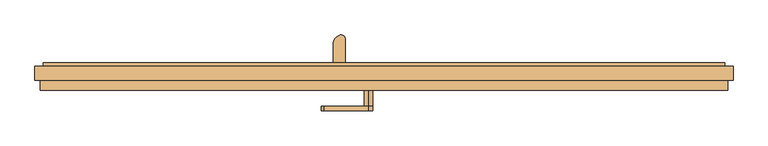
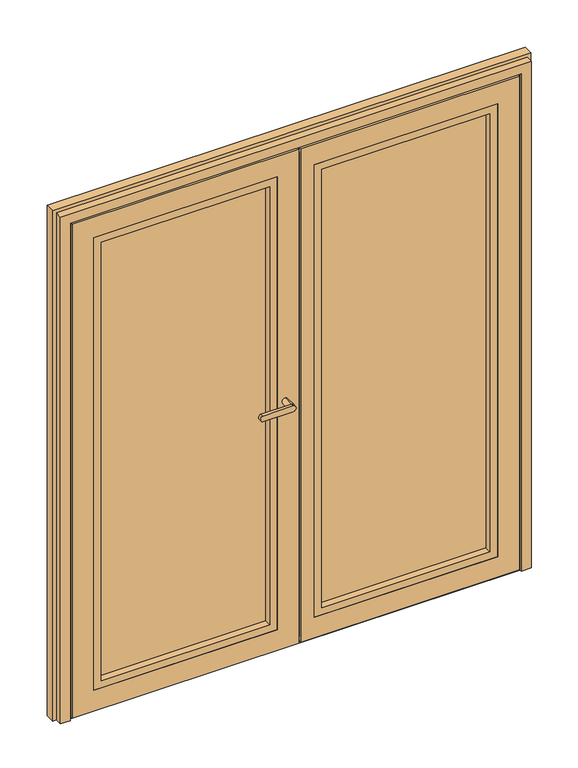
"""IFC4 building model written with IfcOpenShell, lengths in millimetres: door geometry, Schueco_FWS_ADS-75-SimplySmart_inw_Family-02 : FWS SI insert unit."""

from ifc_helpers import new_model, si_unit, point, frame, frame_2d, origin, place, context, project, spatial, polyline, circle_curve, ellipse_curve, trimmed, segment, composite_curve, outline, extrude, faceted_brep, source, transform, mapped, element, save
from ifc_brep_helpers import plane_surface, cylinder_surface, extruded_surface, advanced_brep


def door_de44d966(model_context):
    return source(origin(), model_context, "Body", "SolidModel", [
        faceted_brep([(893.0, -57.5000065, 8.0), (893.0, -57.5000065, 2093.0), (893.0, -66.0002823, 2093.0), (893.0, -66.0002823, 8.0), (19.5, -66.0002823, 8.0), (19.5, -57.5000065, 8.0), (19.5, -57.5000065, 27.0), (874.0, -57.5000065, 27.0), (874.0, -57.5000065, 2074.0), (19.5, -57.5000065, 2074.0), (19.5, -57.5000065, 2093.0), (19.5, -66.0002823, 2093.0), (74.5, -66.0002823, 95.0), (74.5, -66.0002823, 2006.0), (806.0, -66.0002823, 2006.0), (806.0, -66.0002823, 95.0), (806.0, 0.4997603, 2006.0), (806.0, 0.4997603, 95.0), (74.5, 0.4997603, 95.0), (74.5, 0.4997603, 2006.0), (106.5, 0.4997603, 127.0), (106.5, 0.4997603, 1974.0), (774.0, 0.4997603, 1974.0), (774.0, 0.4997603, 127.0), (774.0, 8.9997177, 1974.0), (774.0, 8.9997177, 127.0), (106.5, 8.9997177, 127.0), (106.5, 8.9997177, 1974.0), (861.0, 8.9997177, 40.0), (-12.5, 8.9997177, 40.0), (-12.5, 8.9997177, 2061.0), (861.0, 8.9997177, 2061.0), (861.0, 0.4997603, 2061.0), (861.0, 0.4997603, 40.0), (6.5, 0.4997603, 40.0), (-12.5, 0.4997603, 40.0), (6.5, 0.4997603, 27.0), (6.5, 0.4997603, 2061.0), (6.5, 0.4997603, 2074.0), (874.0, 0.4997603, 2074.0), (874.0, 0.4997603, 27.0), (6.5, -57.5000065, 27.0), (6.5, -57.5000065, 2074.0), (-12.5, 0.4997603, 2061.0)], [[[0, 1, 2, 3]], [[3, 4, 5, 0]], [[0, 5, 6, 7, 8, 9, 10, 1]], [[2, 11, 4, 3], [12, 13, 14, 15]], [[15, 14, 16, 17]], [[17, 18, 12, 15]], [[18, 19, 13, 12]], [[17, 16, 19, 18], [20, 21, 22, 23]], [[23, 22, 24, 25]], [[25, 26, 20, 23]], [[26, 27, 21, 20]], [[28, 29, 30, 31], [25, 24, 27, 26]], [[28, 31, 32, 33]], [[33, 34, 35, 29, 28]], [[36, 34, 33, 32, 37, 38, 39, 40]], [[40, 39, 8, 7]], [[7, 6, 41, 36, 40]], [[41, 42, 38, 37, 34, 36]], [[1, 10, 11, 2]], [[19, 16, 14, 13]], [[27, 24, 22, 21]], [[31, 30, 43, 37, 32]], [[42, 9, 8, 39, 38]], [[6, 5, 4, 11, 10, 9]], [[35, 43, 30, 29]], [[35, 34, 37, 43]], [[9, 42, 41, 6]]]),
        extrude(outline(polyline([(95.0, 74.5), (95.0, 806.0), (2006.0, 806.0), (2006.0, 74.5), (95.0, 74.5)]), holes=[polyline([(125.0, 776.0), (125.0, 104.5), (1976.0, 104.5), (1976.0, 776.0), (125.0, 776.0)])]), frame((0.0, -66.0002823, 0.0), z_axis=(0.0, 1.0, 0.0), x_axis=(0.0, 0.0, 1.0)), (0.0, 0.0, 1.0), 28.5000426),
        extrude(outline(polyline([(74.5, -37.5002397), (74.5, 0.4997603), (806.0, 0.4997603), (806.0, -37.5002397), (74.5, -37.5002397)])), frame((0.0, 0.0, 95.0), z_axis=(0.0, 0.0, 1.0), x_axis=(1.0, 0.0, 0.0)), (0.0, 0.0, 1.0), 1911.0),
        extrude(outline(polyline([(861.0, 0.4997603), (-12.5, 0.4997603), (-12.5, 8.9997177), (861.0, 8.9997177), (861.0, 0.4997603)])), frame((0.0, 0.0, 27.0), z_axis=(0.0, 0.0, 1.0), x_axis=(1.0, 0.0, 0.0)), (0.0, 0.0, 1.0), 13.0),
        extrude(outline(composite_curve([segment(polyline([(-139.1673236, 8.9997177), (-139.1673236, 59.1618682)]), True, "CONTINUOUS"), segment(trimmed(circle_curve(frame_2d((-111.9889059, 59.1618682)), 27.1784177), [point((-139.1673236, 59.1618682))], [point((-121.5260015, 84.6120194))], False, "CARTESIAN"), True, "CONTINUOUS"), segment(trimmed(circle_curve(frame_2d((-117.4485005, 73.7310321)), 11.6198924), [point((-121.5260015, 84.6120194))], [point((-105.8286081, 73.7310321))], False, "CARTESIAN"), True, "CONTINUOUS"), segment(polyline([(-105.8286081, 73.7310321), (-105.8286081, 8.9997177), (-139.1673236, 8.9997177)]), True, "CONTINUOUS")], self_intersect=False)), frame((0.0, 0.0, 2036.9340013), z_axis=(0.0, 0.0, 1.0), x_axis=(1.0, 0.0, 0.0)), (0.0, 0.0, 1.0), 4.0),
        extrude(outline(polyline([(-139.1673236, 12.9997177), (-105.8286081, 12.9997177), (-105.8286081, 8.9997177), (-139.1673236, 8.9997177), (-139.1673236, 12.9997177)])), frame((0.0, 0.0, 2006.9340013), z_axis=(0.0, 0.0, 1.0), x_axis=(1.0, 0.0, 0.0)), (0.0, 0.0, 1.0), 30.0),
        extrude(outline(polyline([(-139.1673236, 12.9997177), (-105.8286081, 12.9997177), (-105.8286081, 8.9997177), (-139.1673236, 8.9997177), (-139.1673236, 12.9997177)])), frame((0.0, 0.0, 56.9340013), z_axis=(0.0, 0.0, 1.0), x_axis=(1.0, 0.0, 0.0)), (0.0, 0.0, 1.0), 30.0),
        extrude(outline(composite_curve([segment(polyline([(-139.1673236, 8.9997177), (-139.1673236, 59.1618682)]), True, "CONTINUOUS"), segment(trimmed(circle_curve(frame_2d((-111.9889059, 59.1618682)), 27.1784177), [point((-139.1673236, 59.1618682))], [point((-121.5260015, 84.6120194))], False, "CARTESIAN"), True, "CONTINUOUS"), segment(trimmed(circle_curve(frame_2d((-117.4485005, 73.7310321)), 11.6198924), [point((-121.5260015, 84.6120194))], [point((-105.8286081, 73.7310321))], False, "CARTESIAN"), True, "CONTINUOUS"), segment(polyline([(-105.8286081, 73.7310321), (-105.8286081, 8.9997177), (-139.1673236, 8.9997177)]), True, "CONTINUOUS")], self_intersect=False)), frame((0.0, 0.0, 52.9340013), z_axis=(0.0, 0.0, 1.0), x_axis=(1.0, 0.0, 0.0)), (0.0, 0.0, 1.0), 4.0),
        advanced_brep(
        [(-109.782924, 57.5977179, 2036.9340013), (-135.217076, 72.2821425, 2036.9340013), (-109.782924, 57.5977179, 56.9340013), (-135.217076, 72.2821425, 56.9340013)],
        [
            (0, 1, ellipse_curve(frame((-122.5, 64.9399302, 2036.9340013), z_axis=(0.0, 0.0, 1.0000000000000002), x_axis=(0.5000002582658958, 0.866025254674503, 0.0)), 21.5840887, 14.6844171)),
            (1, 0, ellipse_curve(frame((-122.5, 64.9399302, 2036.9340013), z_axis=(0.0, 0.0, 1.0000000000000002), x_axis=(0.5000002582658958, 0.866025254674503, 0.0)), 21.5840887, 14.6844171)),
            (2, 3, ellipse_curve(frame((-122.5, 64.9399302, 56.9340013), z_axis=(0.0, 0.0, -1.0000000000000002), x_axis=(-0.866025254674503, 0.5000002582658958, 0.0)), 14.6844171, 21.5840887)),
            (3, 2, ellipse_curve(frame((-122.5, 64.9399302, 56.9340013), z_axis=(0.0, 0.0, -1.0000000000000002), x_axis=(-0.866025254674503, 0.5000002582658958, 0.0)), 14.6844171, 21.5840887)),
            (0, 2),
            (3, 1),
        ],
        [
            plane_surface(frame((-135.217076, 72.2821425, 2036.9340013), z_axis=(0.0, 0.0, 1.0000000000000002), x_axis=(0.5000002582658958, 0.866025254674503, 0.0))),
            plane_surface(frame((-135.217076, 72.2821425, 56.9340013), z_axis=(0.0, 0.0, -1.0000000000000002), x_axis=(-0.5000002582658958, -0.866025254674503, 0.0))),
            extruded_surface(trimmed(ellipse_curve(frame((-122.5, 64.9399302, 56.9340013), z_axis=(0.0, 0.0, -1.0000000000000002), x_axis=(-0.866025254674503, 0.5000002582658958, 0.0)), 14.6844171, 21.5840887), [point((-135.217076, 72.2821425, 56.9340013))], [point((-109.782924, 57.5977179, 56.9340013))], True, "CARTESIAN"), (0.0, 0.0, -1980.0), 1980.0),
            extruded_surface(trimmed(ellipse_curve(frame((-122.5, 64.9399302, 56.9340013), z_axis=(0.0, 0.0, -1.0000000000000002), x_axis=(-0.866025254674503, 0.5000002582658958, 0.0)), 14.6844171, 21.5840887), [point((-109.782924, 57.5977179, 56.9340013))], [point((-135.217076, 72.2821425, 56.9340013))], True, "CARTESIAN"), (0.0, 0.0, -1980.0), 1980.0),
        ],
        [
            (0, [[1, 2]]),
            (1, [[3, 4]]),
            (2, [[5, -4, 6, -1]]),
            (3, [[-6, -3, -5, -2]]),
        ],
    ),
        advanced_brep(
        [(-42.5, -122.0002518, 1038.0113692), (-42.5, -122.0002518, 1061.9886308), (-164.1617926, -122.0002518, 1061.9886308), (-164.1617926, -122.0002518, 1038.0113692), (-42.5, -109.5001648, 1061.9886308), (-42.5, -109.5001648, 1038.0113692), (-164.1617926, -109.5001648, 1038.0113692), (-164.1617926, -109.5001648, 1061.9886308), (-42.5, -66.0002823, 1038.0113692), (-42.5, -66.0002823, 1061.9886308)],
        [
            (0, 1, circle_curve(frame((-42.5, -122.0002518, 1050.0), z_axis=(0.0, -1.0, 0.0), x_axis=(0.0, 0.0, 1.0)), 11.9886308)),
            (1, 2),
            (2, 3, ellipse_curve(frame((-164.1617926, -122.0002518, 1050.0), z_axis=(0.0, -1.0, 0.0), x_axis=(0.0, 0.0, -1.0)), 11.9886308, 7.9050795)),
            (3, 0),
            (4, 5, circle_curve(frame((-42.5, -109.5001648, 1050.0), z_axis=(0.0, -1.0, 0.0), x_axis=(0.0, 0.0, 1.0)), 11.9886308)),
            (5, 6),
            (6, 7, ellipse_curve(frame((-164.1617926, -109.5001648, 1050.0), z_axis=(0.0, 1.0, 0.0), x_axis=(0.0, 0.0, -1.0)), 11.9886308, 7.9050795)),
            (7, 4),
            (3, 6),
            (5, 0),
            (2, 7),
            (1, 4),
            (5, 4, circle_curve(frame((-42.5, -109.5001648, 1050.0), z_axis=(0.0, -1.0, 0.0), x_axis=(0.0, 0.0, 1.0)), 11.9886308)),
            (8, 9, circle_curve(frame((-42.5, -66.0002823, 1050.0), z_axis=(0.0, 1.0, 0.0), x_axis=(0.0, 0.0, 1.0)), 11.9886308)),
            (9, 8, circle_curve(frame((-42.5, -66.0002823, 1050.0), z_axis=(0.0, 1.0, 0.0), x_axis=(0.0, 0.0, 1.0)), 11.9886308)),
            (8, 5),
            (4, 9),
        ],
        [
            plane_surface(frame((-164.1617926, -122.0002518, 1038.0113692), z_axis=(0.0, -1.0, 0.0), x_axis=(-1.0, 0.0, 0.0))),
            plane_surface(frame((-164.1617926, -109.5001648, 1038.0113692), z_axis=(0.0, 1.0, 0.0), x_axis=(1.0, 0.0, 0.0))),
            plane_surface(frame((-42.5, -122.0002518, 1038.0113692), z_axis=(0.0, 0.0, -1.0), x_axis=(0.0, 1.0, 0.0))),
            extruded_surface(trimmed(ellipse_curve(frame((-164.1617926, -109.5001648, 1050.0), z_axis=(0.0, 1.0, 0.0), x_axis=(0.0, 0.0, -1.0)), 11.9886308, 7.9050795), [point((-164.1617926, -109.5001648, 1038.0113692))], [point((-164.1617926, -109.5001648, 1061.9886308))], True, "CARTESIAN"), (0.0, 12.500086999999994, 0.0), 12.500086999999994),
            plane_surface(frame((-164.1617926, -122.0002518, 1061.9886308), z_axis=(0.0, 0.0, 1.0), x_axis=(0.0, 1.0, 0.0))),
            cylinder_surface(frame((-42.5, -109.5001648, 1050.0), z_axis=(0.0, -1.0, 0.0), x_axis=(0.0, 0.0, 1.0)), 11.9886308),
            plane_surface(frame((-42.5, -66.0002823, 1061.9886308), z_axis=(0.0, 1.0, 0.0), x_axis=(-1.0, 0.0, 0.0))),
            cylinder_surface(frame((-42.5, -66.0002823, 1050.0), z_axis=(0.0, -1.0, 0.0), x_axis=(0.0, 0.0, 1.0)), 11.9886308),
        ],
        [
            (0, [[1, 2, 3, 4]]),
            (1, [[5, 6, 7, 8]]),
            (2, [[9, -6, 10, -4]]),
            (3, [[11, -7, -9, -3]]),
            (4, [[12, -8, -11, -2]]),
            (5, [[-10, 13, -12, -1]]),
            (6, [[14, 15]]),
            (7, [[16, -5, 17, -14]]),
            (7, [[-17, -13, -16, -15]]),
        ],
    ),
        faceted_brep([(-893.0, -57.5000065, 8.0), (-893.0, -66.0002823, 8.0), (-893.0, -66.0002823, 2093.0), (-893.0, -57.5000065, 2093.0), (12.5, -57.5000065, 8.0), (12.5, -66.0002823, 8.0), (12.5, -57.5000065, 2093.0), (-874.0, -57.5000065, 27.0), (-6.5, -57.5000065, 27.0), (-6.5, -57.5000065, 2074.0), (-874.0, -57.5000065, 2074.0), (12.5, -66.0002823, 2093.0), (-74.5, -66.0002823, 95.0), (-806.0, -66.0002823, 95.0), (-806.0, -66.0002823, 2006.0), (-74.5, -66.0002823, 2006.0), (-806.0, 0.4997603, 95.0), (-806.0, 0.4997603, 2006.0), (-74.5, 0.4997603, 95.0), (-74.5, 0.4997603, 2006.0), (-106.5, 0.4997603, 127.0), (-774.0, 0.4997603, 127.0), (-774.0, 0.4997603, 1974.0), (-106.5, 0.4997603, 1974.0), (-774.0, 8.9997177, 127.0), (-774.0, 8.9997177, 1974.0), (-106.5, 8.9997177, 127.0), (-106.5, 8.9997177, 1974.0), (-19.5, 8.9997177, 2061.0), (-19.5, 8.9997177, 40.0), (-22.4962682, 8.9997177, 40.0), (-861.0, 8.9997177, 40.0), (-861.0, 8.9997177, 2061.0), (-22.4962682, 8.9997177, 2061.0), (-861.0, 0.4997603, 40.0), (-861.0, 0.4997603, 2061.0), (-19.5, 0.4997603, 40.0), (-22.4962682, 0.4997603, 40.0), (-19.5, 0.4997603, 2061.0), (-6.5, 0.4997603, 27.0), (-874.0, 0.4997603, 27.0), (-874.0, 0.4997603, 2074.0), (-6.5, 0.4997603, 2074.0), (-22.4962682, 0.4997603, 2061.0)], [[[0, 1, 2, 3]], [[1, 0, 4, 5]], [[4, 0, 3, 6], [7, 8, 9, 10]], [[5, 4, 6, 11]], [[1, 5, 11, 2], [12, 13, 14, 15]], [[13, 16, 17, 14]], [[16, 13, 12, 18]], [[18, 12, 15, 19]], [[16, 18, 19, 17], [20, 21, 22, 23]], [[21, 24, 25, 22]], [[24, 21, 20, 26]], [[26, 20, 23, 27]], [[28, 29, 30, 31, 32, 33], [24, 26, 27, 25]], [[31, 34, 35, 32]], [[34, 31, 30, 29, 36, 37]], [[36, 29, 28, 38]], [[39, 40, 41, 42], [36, 38, 43, 35, 34, 37]], [[40, 7, 10, 41]], [[7, 40, 39, 8]], [[8, 39, 42, 9]], [[11, 6, 3, 2]], [[19, 15, 14, 17]], [[27, 23, 22, 25]], [[38, 28, 33, 32, 35, 43]], [[9, 42, 41, 10]]]),
        extrude(outline(polyline([(95.0, -74.5), (2006.0, -74.5), (2006.0, -806.0), (95.0, -806.0), (95.0, -74.5)]), holes=[polyline([(125.0, -776.0), (1976.0, -776.0), (1976.0, -104.5), (125.0, -104.5), (125.0, -776.0)])]), frame((0.0, -66.0002823, 0.0), z_axis=(0.0, 1.0, 0.0), x_axis=(0.0, 0.0, 1.0)), (0.0, 0.0, 1.0), 28.5000426),
        extrude(outline(polyline([(-74.5, -37.5002397), (-806.0, -37.5002397), (-806.0, 0.4997603), (-74.5, 0.4997603), (-74.5, -37.5002397)])), frame((0.0, 0.0, 95.0), z_axis=(0.0, 0.0, 1.0), x_axis=(1.0, 0.0, 0.0)), (0.0, 0.0, 1.0), 1911.0),
        extrude(outline(polyline([(-861.0, 0.4997603), (-861.0, 8.9997177), (-19.5, 8.9997177), (-19.5, 0.4997603), (-861.0, 0.4997603)])), frame((0.0, 0.0, 27.0), z_axis=(0.0, 0.0, 1.0), x_axis=(1.0, 0.0, 0.0)), (0.0, 0.0, 1.0), 13.0),
        faceted_brep([(930.999943, 8.9997177, 2130.999943), (930.999943, 0.0, 2130.999943), (930.999943, 0.0, 0.0), (930.999943, 8.9997177, 0.0), (-954.0, 0.0, 0.0), (-954.0, 0.0, 2154.0), (954.0, 0.0, 2154.0), (954.0, 0.0, 0.0), (-930.999943, 0.0, 2130.999943), (-930.999943, 0.0, 0.0), (954.0, -38.0, 0.0), (940.0, -38.0, 0.0), (940.0, -66.0002823, 0.0), (899.9999732, -66.0002823, 0.0), (899.9999732, -57.5000065, 0.0), (886.9999732, -57.5000065, 0.0), (886.9999732, 0.4997603, 0.0), (867.9999732, 0.4997603, 0.0), (867.9999732, 8.9997177, 0.0), (-867.9999732, 8.9997177, 0.0), (-930.999943, 8.9997177, 0.0), (-930.999943, 8.9997177, 2130.999943), (867.9999732, 8.9997177, 2067.9999732), (-867.9999732, 8.9997177, 2067.9999732), (899.9999732, -66.0002823, 2099.9999732), (899.9999732, -57.5000065, 2099.9999732), (-899.9999732, -57.5000065, 0.0), (-886.9999732, -57.5000065, 0.0), (-886.9999732, -57.5000065, 2086.9999732), (886.9999732, -57.5000065, 2086.9999732), (-899.9999732, -57.5000065, 2099.9999732), (-940.0, -66.0002823, 0.0), (-899.9999732, -66.0002823, 0.0), (-899.9999732, -66.0002823, 2099.9999732), (940.0, -66.0002823, 2140.0), (-940.0, -66.0002823, 2140.0), (940.0, -38.0, 2140.0), (-954.0, -38.0, 0.0), (-940.0, -38.0, 0.0), (-940.0, -38.0, 2140.0), (954.0, -38.0, 2154.0), (-954.0, -38.0, 2154.0), (-867.9999732, 0.4997603, 0.0), (-886.9999732, 0.4997603, 0.0), (867.9999732, 0.4997603, 2067.9999732), (-867.9999732, 0.4997603, 2067.9999732), (886.9999732, 0.4997603, 2086.9999732), (-886.9999732, 0.4997603, 2086.9999732)], [[[0, 1, 2, 3]], [[4, 5, 6, 7, 2, 1, 8, 9]], [[3, 2, 7, 10, 11, 12, 13, 14, 15, 16, 17, 18]], [[19, 20, 21, 0, 3, 18, 22, 23]], [[24, 25, 14, 13]], [[26, 27, 28, 29, 15, 14, 25, 30]], [[31, 32, 33, 24, 13, 12, 34, 35]], [[34, 12, 11, 36]], [[37, 38, 39, 36, 11, 10, 40, 41]], [[4, 9, 20, 19, 42, 43, 27, 26, 32, 31, 38, 37]], [[20, 9, 8, 21]], [[18, 17, 44, 22]], [[42, 19, 23, 45]], [[32, 26, 30, 33]], [[31, 35, 39, 38]], [[4, 37, 41, 5]], [[6, 40, 10, 7]], [[43, 42, 45, 44, 17, 16, 46, 47]], [[16, 15, 29, 46]], [[27, 43, 47, 28]], [[21, 8, 1, 0]], [[33, 30, 25, 24]], [[35, 34, 36, 39]], [[23, 22, 44, 45]], [[5, 41, 40, 6]], [[47, 46, 29, 28]]]),
        extrude(outline(polyline([(8.9997177, 13.2857074), (8.9997177, 0.0), (-57.5000065, 0.0), (-57.5000065, 14.1033166), (-13.0000038, 14.1033166), (-13.0000038, 20.0), (-10.5000038, 20.0), (8.9997177, 13.2857074)])), frame((-888.5, 0.0, 0.0), z_axis=(1.0, 0.0, 0.0), x_axis=(0.0, 1.0, 0.0)), (0.0, 0.0, 1.0), 1776.9999732),
    ])


if __name__ == "__main__":
    model = new_model("IFC4")
    model_context = context("Model", 3, world=origin())
    ifc_project = project(units=[si_unit("LENGTHUNIT", "METRE", prefix="MILLI")], contexts=[model_context])
    site = spatial("IfcSite", under=ifc_project)
    building = spatial("IfcBuilding", under=site)
    placement = place(None, origin())
    door_shape = door_de44d966(model_context)
    element("IfcDoor", 1, ObjectType="Schueco_FWS_ADS-75-SimplySmart_inw_Family-02 : FWS SI insert unit", at=placement, inside=building, context=model_context, shape_type="MappedRepresentation", body=[
        mapped(door_shape, transform((0.0, 0.0, 0.0), x_axis=(1.0, 0.0, 0.0), y_axis=(0.0, 1.0, 0.0), z_axis=(0.0, 0.0, 1.0))),
    ])
    save(model, "model.ifc")

# Revit data of these elements
# Type "Schueco_FWS_ADS-75-SimplySmart_inw_Family-02 : FWS SI insert unit"
#   Type Mark = "54"
#   __NOTE__ = "Data describes the optimum values of the entire system. The properites of a selected design option have to be determined on an individual basis!"
#   Wind load resistance = "Class C3"
#   Watertightness = "Class E750"
#   Thermal insulation = "Uf = 1.6 W/(m²K)"
#   Sound insulation = "..."
#   Schueco thermal insulation standard = "Highly thermally insulated"
#   Opening type = "Inward-opening, Flush-fitted"
#   Model = "Schueco ADS 75 SimplySmart"
#   Mechanical loading = "..."
#   Maximum leaf width in mm = "1400"
#   Maximum leaf weight in kg = "200"
#   Maximum leaf height in mm = "3000"
#   Material = "Aluminium"
#   Long term functionality = "..."
#   Construction Type = "Door, double-leaf, inward-opening"
#   Manufacturer = "Schueco International KG"
#   Glazing data = "Triple glazing 38mm"
#   Façade insert unit = "yes"
#   Family creation date = "08.2017"
#   Description = "Schueco Aluminium Door System (ADS)"
#   Burglar resistance = "Class RC 2"
#   Areas of use = "Public buildings, Residential buildings, Side entrance"
#   Analytic Construction = "<None>"
#   Air permeability = "Class 4"
#   Width [instance default] = 962.602 mm
#   Leaf opening angle [instance default] = 0.00°
#   IOf_T = 38 mm
#   Height [instance default] = 2117.739 mm
#   Glazing area [instance default] = 0.705468 m²
#   F2_W [instance default] = 481.301 mm
#   F1_W [instance default] = 481.301 mm
#   Distance from bottom to handles [instance default] = 1050 mm
#   Clear opening width [instance default] = 790.602 mm
#   Active leaf width = 1100 mm
#   Standard threshold = yes
#   Low level threshold = no
#   Handles = yes
#   All fields of identical width = yes
#   Glass = none
#   Frame = Alu
#   Fittings = none
# Element 1 (IfcDoor, "Schueco_FWS_ADS-75-SimplySmart_inw_Family-02 : FWS SI insert unit")
#   Width = 1908 mm
#   Height = 2154 mm
#   Glazing area = 2.46575 m²
#   F2_W = 954 mm
#   F1_W = 954 mm
#   Clear opening width = 1736 mm
#   Materials on its faces: "Alu", "Glass"
# Materials
#   "Alu": class "Glas", colour RGB 140 140 140, transparency 0
#   "Glass": class "Glass", colour RGB 128 128 255, transparency 0.75, Description = "Soda Lime Glass", Cost = 0
